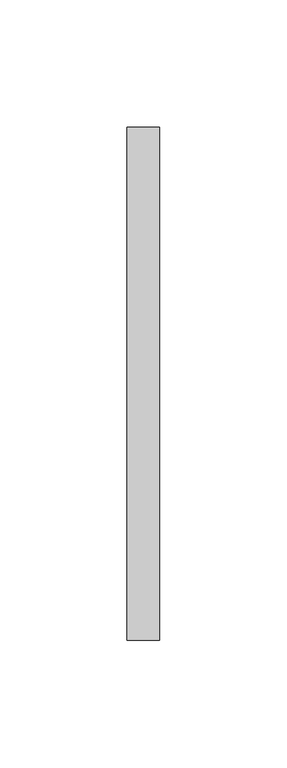
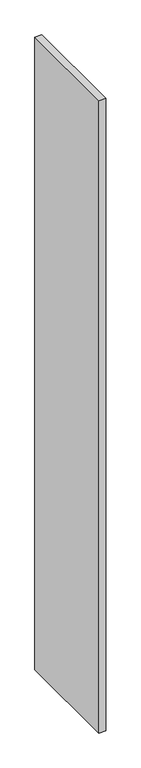
"""IFC4 building model written with IfcOpenShell, lengths in millimetres: proxy geometry, Inner panel:Inner panel:1:Inner panel:1 : Inner panel:Inner panel:300324:300043:Inner panel:1:Inner panel:1 : Inner panel:Inner panel:300324:300043 : Inner panel:Inner panel:1:Inner panel:1 : Inner panel:Inner panel:300324:300043:39 : Inner panel:Inner panel:1:Inner panel:1 : Inner panel:Inner panel:300324:300043:Inner panel:1:Inner panel:1 : Inner panel:Inner panel:300324:300043 : Inner panel:Inner panel:1:Inner panel:1 : Inner panel:Inner panel:300324:300043:300031."""

from ifc_helpers import new_model, si_unit, frame, origin, place, context, project, spatial, polyline, outline, extrude, source, transform, mapped, element, save


def generic_models_419a4776(model_context):
    return source(origin(), model_context, "Body", "SweptSolid", [
        extrude(outline(polyline([(560365.6617239, -579000.6913841), (560352.9617239, -579000.6913841), (560352.9617239, -578799.4515458), (560365.6617239, -578799.4515458), (560365.6617239, -579000.6913841)])), frame((0.0, 0.0, 3721.1), z_axis=(0.0, 0.0, 1.0), x_axis=(1.0, 0.0, 0.0)), (0.0, 0.0, 1.0), 1219.2),
    ])


if __name__ == "__main__":
    model = new_model("IFC4")
    model_context = context("Model", 3, world=origin())
    ifc_project = project(units=[si_unit("LENGTHUNIT", "METRE", prefix="MILLI")], contexts=[model_context])
    site = spatial("IfcSite", under=ifc_project)
    building = spatial("IfcBuilding", under=site)
    placement = place(None, origin())
    generic_models_shape = generic_models_419a4776(model_context)
    element("IfcBuildingElementProxy", 1, Name="Inner panel:Inner panel:1:Inner panel:1 : Inner panel:Inner panel:300324:300043:Inner panel:1:Inner panel:1 : Inner panel:Inner panel:300324:300043 : Inner panel:Inner panel:1:Inner panel:1 : Inner panel:Inner panel:300324:300043:39 : Inner panel:Inner panel:1:Inner panel:1 : Inner panel:Inner panel:300324:300043:Inner panel:1:Inner panel:1 : Inner panel:Inner panel:300324:300043 : Inner panel:Inner panel:1:Inner panel:1 : Inner panel:Inner panel:300324:300043:300031", ObjectType="Inner panel:Inner panel:1:Inner panel:1 : Inner panel:Inner panel:300324:300043:Inner panel:1:Inner panel:1 : Inner panel:Inner panel:300324:300043 : Inner panel:Inner panel:1:Inner panel:1 : Inner panel:Inner panel:300324:300043:39 : Inner panel:Inner panel:1:Inner panel:1 : Inner panel:Inner panel:300324:300043:Inner panel:1:Inner panel:1 : Inner panel:Inner panel:300324:300043 : Inner panel:Inner panel:1:Inner panel:1 : Inner panel:Inner panel:300324:300043:300031", at=placement, inside=building, context=model_context, shape_type="MappedRepresentation", body=[
        mapped(generic_models_shape, transform((0.0, 0.0, 0.0), x_axis=(1.0, 0.0, 0.0), y_axis=(0.0, 1.0, 0.0), z_axis=(0.0, 0.0, 1.0))),
    ])
    save(model, "model.ifc")

# Revit data of these elements
# Type "Inner panel:Inner panel:1:Inner panel:1 : Inner panel:Inner panel:300324:300043:Inner panel:1:Inner panel:1 : Inner panel:Inner panel:300324:300043 : Inner panel:Inner panel:1:Inner panel:1 : Inner panel:Inner panel:300324:300043:39 : Inner panel:Inner panel:1:Inner panel:1 : Inner panel:Inner panel:300324:300043:Inner panel:1:Inner panel:1 : Inner panel:Inner panel:300324:300043 : Inner panel:Inner panel:1:Inner panel:1 : Inner panel:Inner panel:300324:300043:300031"
#   NameOverride = "Inner panel:Inner panel:1:Inner panel:1 : Inner panel:Inner panel:300324:300043:Inner panel:1:Inner panel:1 : Inner panel:Inner panel:300324:300043 : Inner panel:Inner panel:1:Inner panel:1 : Inner panel:Inner panel:300324:300043:300031"
#   ObjectTypeOverride = "Inner panel:1:Inner panel:1 : Inner panel:Inner panel:300324:300043 : Inner panel:Inner panel:1:Inner panel:1 : Inner panel:Inner panel:300324:300043"
#   Reference = "Inner panel"
#   Tag = "300031"
# Element 1 (IfcBuildingElementProxy, "Inner panel:Inner panel:1:Inner panel:1 : Inner panel:Inner panel:300324:300043:Inner panel:1:Inner panel:1 : Inner panel:Inner panel:300324:300043 : Inner panel:Inner panel:1:Inner panel:1 : Inner panel:Inner panel:300324:300043:39 : Inner panel:Inner panel:1:Inner panel:1 : Inner panel:Inner panel:300324:300043:Inner panel:1:Inner panel:1 : Inner panel:Inner panel:300324:300043 : Inner panel:Inner panel:1:Inner panel:1 : Inner panel:Inner panel:300324:300043:300031")
#   Materials on its faces: "1/2\" FIBERGLASS MAT GYPSUM PANELS"
# Materials
#   "1/2\" FIBERGLASS MAT GYPSUM PANELS": class "Generic", colour RGB 171 170 168, transparency 0, Description = "Gypsum Wall Board", Cost = 0
